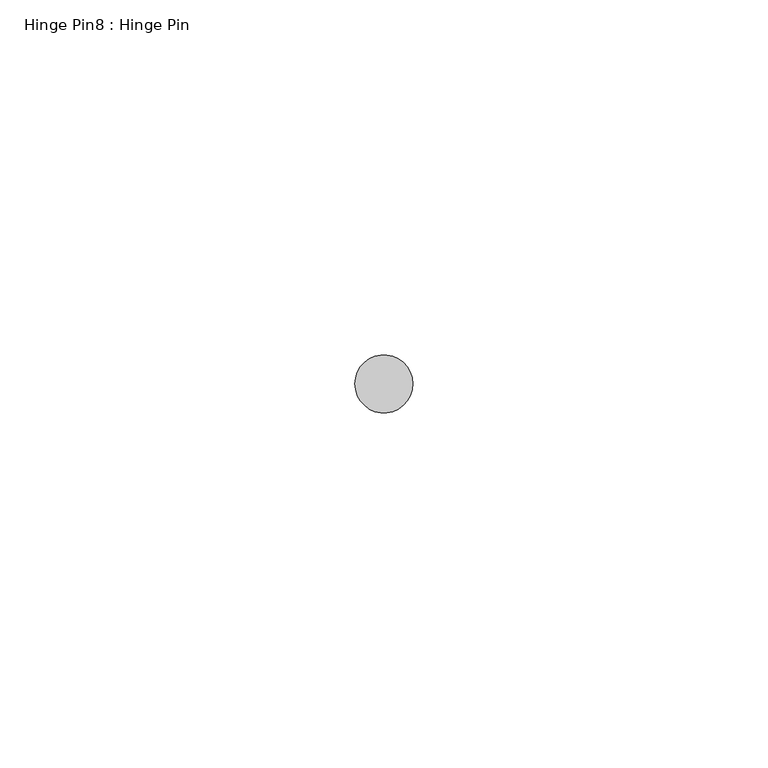
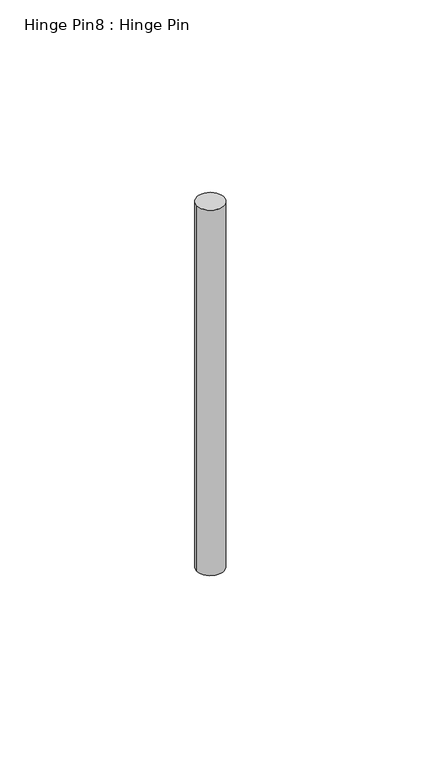
"""IFC4 building model written with IfcOpenShell, lengths in millimetres: proxy geometry, Hinge Pin8 : Hinge Pin."""

from ifc_helpers import new_model, si_unit, point, frame, frame_2d, origin, place, context, project, spatial, circle_curve, trimmed, segment, composite_curve, outline, extrude, source, transform, mapped, element, save


def hinge_pin8_hinge_pin_bc855f33(model_context):
    return source(origin(), model_context, "Body", "SweptSolid", [
        extrude(outline(composite_curve([segment(trimmed(circle_curve(frame_2d((587319.1320739, -534100.7049841)), 4.0894), [point((587315.0426739, -534100.7049841))], [point((587323.2214739, -534100.7049841))], False, "CARTESIAN"), True, "CONTINUOUS"), segment(trimmed(circle_curve(frame_2d((587319.1320739, -534100.7049841)), 4.0894), [point((587323.2214739, -534100.7049841))], [point((587315.0426739, -534100.7049841))], False, "CARTESIAN"), True, "CONTINUOUS")], self_intersect=False)), frame((0.0, 0.0, 1128.5140625), z_axis=(0.0, 0.0, 1.0), x_axis=(1.0, 0.0, 0.0)), (0.0, 0.0, 1.0), 117.871875),
    ])


if __name__ == "__main__":
    model = new_model("IFC4")
    model_context = context("Model", 3, world=origin())
    ifc_project = project(units=[si_unit("LENGTHUNIT", "METRE", prefix="MILLI")], contexts=[model_context])
    site = spatial("IfcSite", under=ifc_project)
    building = spatial("IfcBuilding", under=site)
    placement = place(None, origin())
    hinge_pin8_hinge_pin_shape = hinge_pin8_hinge_pin_bc855f33(model_context)
    element("IfcBuildingElementProxy", 1, Name="Hinge Pin8 : Hinge Pin", ObjectType="Hinge Pin8 : Hinge Pin", at=placement, inside=building, context=model_context, shape_type="MappedRepresentation", body=[
        mapped(hinge_pin8_hinge_pin_shape, transform((0.0, 0.0, 0.0), x_axis=(1.0, 0.0, 0.0), y_axis=(0.0, 1.0, 0.0), z_axis=(0.0, 0.0, 1.0))),
    ])
    save(model, "model.ifc")

# Revit data of these elements
# Element 1 (IfcBuildingElementProxy, "Hinge Pin8 : Hinge Pin")
#   Materials on its faces: "6\"X6\" WELD-ON STL BUTT HINGE"
# Materials
#   "6\"X6\" WELD-ON STL BUTT HINGE": class "Metal", colour RGB 189 187 185, transparency 0, Description = "Carbon steel", Cost = 0
